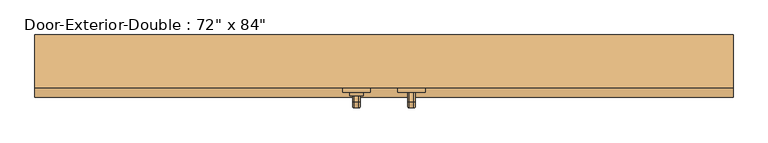
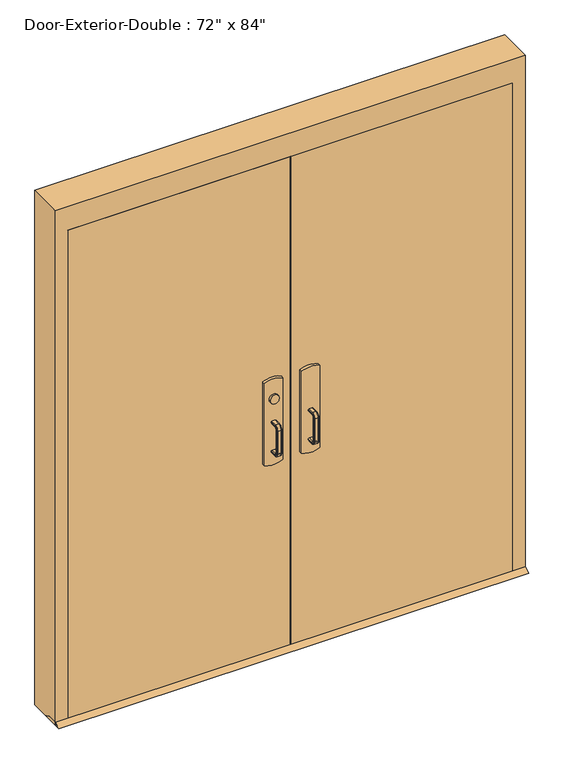
"""IFC4 building model written with IfcOpenShell, lengths in millimetres: door geometry."""

from ifc_helpers import new_model, si_unit, point, frame, frame_2d, origin, place, context, project, spatial, polyline, circle_curve, ellipse_curve, trimmed, segment, composite_curve, outline, extrude, faceted_brep, source, transform, mapped, element, save
from ifc_brep_helpers import plane_surface, cylinder_surface, revolved_surface, advanced_brep


def door_c6cb3189(model_context):
    return source(origin(), model_context, "Body", "SolidModel", [
        extrude(outline(polyline([(-575.7333333, 12.7), (-76.2, 12.7), (-76.2, 6.35), (-575.7333333, 6.35), (-575.7333333, 12.7)])), frame((0.0, 0.0, 990.6), z_axis=(0.0, 0.0, 1.0), x_axis=(1.0, 0.0, 0.0)), (0.0, 0.0, 1.0), 50.8),
        advanced_brep(
        [(-12.7, 6.35, 1041.4), (-12.7, 6.35, 990.6), (-76.2, 6.35, 990.6), (-825.5, 6.35, 990.6), (-825.5, 6.35, 1041.4), (-76.2, 6.35, 1041.4), (-825.5, -25.4, 1041.4), (-825.5, -25.4, 990.6), (-76.2, -25.4, 990.6), (-76.2, -25.4, 927.1), (-57.15, -25.4, 908.05), (-31.75, -25.4, 908.05), (-12.7, -25.4, 927.1), (-12.7, -25.4, 1104.9), (-31.75, -25.4, 1123.95), (-57.15, -25.4, 1123.95), (-76.2, -25.4, 1104.9), (-76.2, -25.4, 1041.4), (-76.2, 3.1747533, 1041.4), (-12.7, 3.1747533, 1041.4), (-12.7, -1.8354269, 1104.9), (-12.7, -1.8354269, 927.1), (-12.7, 3.1747533, 990.6), (-76.2, 3.1747533, 990.6), (-76.2, -1.8354269, 1104.9), (-76.2, -1.8354269, 927.1), (-31.75, -3.338481, 1123.95), (-57.15, -3.338481, 1123.95), (-57.15, -3.338481, 908.05), (-31.75, -3.338481, 908.05)],
        [
            (0, 1),
            (1, 2),
            (2, 3),
            (3, 4),
            (4, 5),
            (5, 0),
            (6, 7),
            (7, 8),
            (8, 9),
            (9, 10, circle_curve(frame((-57.15, -25.4, 927.1), z_axis=(0.0, -1.0, 0.0), x_axis=(-1.0, 0.0, 0.0)), 19.05)),
            (10, 11),
            (11, 12, circle_curve(frame((-31.75, -25.4, 927.1), z_axis=(0.0, -1.0, 0.0), x_axis=(-1.0, 0.0, 0.0)), 19.05)),
            (12, 13),
            (13, 14, circle_curve(frame((-31.75, -25.4, 1104.9), z_axis=(0.0, -1.0, 0.0), x_axis=(-1.0, 0.0, 0.0)), 19.05)),
            (14, 15),
            (15, 16, circle_curve(frame((-57.15, -25.4, 1104.9), z_axis=(0.0, -1.0, 0.0), x_axis=(-1.0, 0.0, 0.0)), 19.05)),
            (16, 17),
            (17, 6),
            (4, 6),
            (17, 18),
            (18, 19),
            (19, 0),
            (19, 20),
            (20, 13),
            (12, 21),
            (21, 22),
            (22, 1),
            (7, 3),
            (22, 23),
            (23, 8),
            (16, 24),
            (24, 18),
            (23, 25),
            (25, 9),
            (14, 26),
            (26, 27),
            (27, 15),
            (10, 28),
            (28, 29),
            (29, 11),
            (25, 28, ellipse_curve(frame((-57.15, -1.8354269, 927.1), z_axis=(0.0, -0.9969018152893365, 0.07865602756830282), x_axis=(0.0, 0.07865602756830208, 0.9969018152893365)), 19.1092038, 19.05)),
            (27, 24, ellipse_curve(frame((-57.15, -1.8354269, 1104.9), z_axis=(0.0, -0.9969018152893376, -0.07865602756828934), x_axis=(0.0, 0.078656027568288, -0.9969018152893377)), 19.1092038, 19.05)),
            (20, 26, ellipse_curve(frame((-31.75, -1.8354269, 1104.9), z_axis=(0.0, -0.9969018152893376, -0.07865602756828934), x_axis=(0.0, 0.078656027568288, -0.9969018152893377)), 19.1092038, 19.05)),
            (29, 21, ellipse_curve(frame((-31.75, -1.8354269, 927.1), z_axis=(0.0, -0.9969018152893365, 0.07865602756830282), x_axis=(0.0, 0.07865602756830208, 0.9969018152893365)), 19.1092038, 19.05)),
        ],
        [
            plane_surface(frame((-12.7, 6.35, 1041.4), z_axis=(0.0, 1.0, 0.0), x_axis=(1.0, 0.0, 0.0))),
            plane_surface(frame((-12.7, -25.4, 1041.4), z_axis=(0.0, -1.0, 0.0), x_axis=(-1.0, 0.0, 0.0))),
            plane_surface(frame((-825.5, 6.35, 1041.4), z_axis=(0.0, 0.0, 1.0), x_axis=(0.0, -1.0, 0.0))),
            plane_surface(frame((-12.7, 6.35, 1041.4), z_axis=(1.0, 0.0, 0.0), x_axis=(0.0, -1.0, 0.0))),
            plane_surface(frame((-12.7, 6.35, 990.6), z_axis=(0.0, 0.0, -1.0), x_axis=(0.0, -1.0, 0.0))),
            plane_surface(frame((-825.5, 6.35, 990.6), z_axis=(-1.0, 0.0, 0.0), x_axis=(0.0, -1.0, 0.0))),
            plane_surface(frame((-76.2, 3.1747533, 927.1), z_axis=(-1.0, 0.0, 0.0), x_axis=(0.0, -1.0, 0.0))),
            plane_surface(frame((-57.15, 3.1747533, 1123.95), z_axis=(0.0, 0.0, 1.0), x_axis=(0.0, -1.0, 0.0))),
            plane_surface(frame((-31.75, 3.1747533, 908.05), z_axis=(0.0, 0.0, -1.0), x_axis=(0.0, -1.0, 0.0))),
            cylinder_surface(frame((-57.15, -25.4, 927.1), z_axis=(0.0, 1.0, 0.0), x_axis=(-1.0, 0.0, 0.0)), 19.05),
            cylinder_surface(frame((-57.15, -25.4, 1104.9), z_axis=(0.0, 1.0, 0.0), x_axis=(-1.0, 0.0, 0.0)), 19.05),
            cylinder_surface(frame((-31.75, -25.4, 1104.9), z_axis=(0.0, 1.0, 0.0), x_axis=(-1.0, 0.0, 0.0)), 19.05),
            cylinder_surface(frame((-31.75, -25.4, 927.1), z_axis=(0.0, 1.0, 0.0), x_axis=(-1.0, 0.0, 0.0)), 19.05),
            plane_surface(frame((-76.2, 3.1747533, 1041.4), z_axis=(0.0, 0.9969018152893376, 0.07865602756828934), x_axis=(1.0, 0.0, 0.0))),
            plane_surface(frame((-76.2, -3.338481, 908.05), z_axis=(0.0, 0.9969018152893365, -0.07865602756830282), x_axis=(1.0, 0.0, 0.0))),
        ],
        [
            (0, [[1, 2, 3, 4, 5, 6]]),
            (1, [[7, 8, 9, 10, 11, 12, 13, 14, 15, 16, 17, 18]]),
            (2, [[19, -18, 20, 21, 22, -6, -5]]),
            (3, [[-1, -22, 23, 24, -13, 25, 26, 27]]),
            (4, [[28, -3, -2, -27, 29, 30, -8]]),
            (5, [[-4, -28, -7, -19]]),
            (6, [[-17, 31, 32, -20]]),
            (6, [[-9, -30, 33, 34]]),
            (7, [[-15, 35, 36, 37]]),
            (8, [[-11, 38, 39, 40]]),
            (9, [[-10, -34, 41, -38]]),
            (10, [[-16, -37, 42, -31]]),
            (11, [[-14, -24, 43, -35]]),
            (12, [[-12, -40, 44, -25]]),
            (13, [[-21, -32, -42, -36, -43, -23]]),
            (14, [[-26, -44, -39, -41, -33, -29]]),
        ],
    ),
        extrude(outline(polyline([(-69.85, 12.7), (-25.4, 12.7), (0.0, 0.0), (-95.25, 0.0), (-69.85, 12.7)])), frame((-965.2, 0.0, 0.0), z_axis=(1.0, 0.0, 0.0), x_axis=(0.0, 1.0, 0.0)), (0.0, 0.0, 1.0), 1930.4),
        extrude(outline(polyline([(575.7333333, 12.7), (575.7333333, 6.35), (76.2, 6.35), (76.2, 12.7), (575.7333333, 12.7)])), frame((0.0, 0.0, 990.6), z_axis=(0.0, 0.0, 1.0), x_axis=(1.0, 0.0, 0.0)), (0.0, 0.0, 1.0), 50.8),
        advanced_brep(
        [(12.7, 6.35, 1041.4), (76.2, 6.35, 1041.4), (825.5, 6.35, 1041.4), (825.5, 6.35, 990.6), (76.2, 6.35, 990.6), (12.7, 6.35, 990.6), (825.5, -25.4, 1041.4), (76.2, -25.4, 1041.4), (76.2, -25.4, 1104.9), (57.15, -25.4, 1123.95), (31.75, -25.4, 1123.95), (12.7, -25.4, 1104.9), (12.7, -25.4, 927.1), (31.75, -25.4, 908.05), (57.15, -25.4, 908.05), (76.2, -25.4, 927.1), (76.2, -25.4, 990.6), (825.5, -25.4, 990.6), (12.7, 3.1747533, 1041.4), (76.2, 3.1747533, 1041.4), (12.7, 3.1747533, 990.6), (12.7, -1.8354269, 927.1), (12.7, -1.8354269, 1104.9), (76.2, 3.1747533, 990.6), (76.2, -1.8354269, 1104.9), (76.2, -1.8354269, 927.1), (57.15, -3.338481, 1123.95), (31.75, -3.338481, 1123.95), (31.75, -3.338481, 908.05), (57.15, -3.338481, 908.05)],
        [
            (0, 1),
            (1, 2),
            (2, 3),
            (3, 4),
            (4, 5),
            (5, 0),
            (6, 7),
            (7, 8),
            (8, 9, circle_curve(frame((57.15, -25.4, 1104.9), z_axis=(0.0, -1.0, 0.0), x_axis=(1.0, 0.0, 0.0)), 19.05)),
            (9, 10),
            (10, 11, circle_curve(frame((31.75, -25.4, 1104.9), z_axis=(0.0, -1.0, 0.0), x_axis=(1.0, 0.0, 0.0)), 19.05)),
            (11, 12),
            (12, 13, circle_curve(frame((31.75, -25.4, 927.1), z_axis=(0.0, -1.0, 0.0), x_axis=(1.0, 0.0, 0.0)), 19.05)),
            (13, 14),
            (14, 15, circle_curve(frame((57.15, -25.4, 927.1), z_axis=(0.0, -1.0, 0.0), x_axis=(1.0, 0.0, 0.0)), 19.05)),
            (15, 16),
            (16, 17),
            (17, 6),
            (0, 18),
            (18, 19),
            (19, 7),
            (6, 2),
            (5, 20),
            (20, 21),
            (21, 12),
            (11, 22),
            (22, 18),
            (16, 23),
            (23, 20),
            (3, 17),
            (19, 24),
            (24, 8),
            (15, 25),
            (25, 23),
            (9, 26),
            (26, 27),
            (27, 10),
            (13, 28),
            (28, 29),
            (29, 14),
            (29, 25, ellipse_curve(frame((57.15, -1.8354269, 927.1), z_axis=(0.0, -0.9969018152893365, 0.07865602756830282), x_axis=(0.0, 0.07865602756830208, 0.9969018152893365)), 19.1092038, 19.05)),
            (24, 26, ellipse_curve(frame((57.15, -1.8354269, 1104.9), z_axis=(0.0, -0.9969018152893376, -0.07865602756828934), x_axis=(0.0, 0.078656027568288, -0.9969018152893377)), 19.1092038, 19.05)),
            (27, 22, ellipse_curve(frame((31.75, -1.8354269, 1104.9), z_axis=(0.0, -0.9969018152893376, -0.07865602756828934), x_axis=(0.0, 0.078656027568288, -0.9969018152893377)), 19.1092038, 19.05)),
            (21, 28, ellipse_curve(frame((31.75, -1.8354269, 927.1), z_axis=(0.0, -0.9969018152893365, 0.07865602756830282), x_axis=(0.0, 0.07865602756830208, 0.9969018152893365)), 19.1092038, 19.05)),
        ],
        [
            plane_surface(frame((12.7, 6.35, 1041.4), z_axis=(0.0, 1.0, 0.0), x_axis=(-1.0, 0.0, 0.0))),
            plane_surface(frame((12.7, -25.4, 1041.4), z_axis=(0.0, -1.0, 0.0), x_axis=(1.0, 0.0, 0.0))),
            plane_surface(frame((825.5, 6.35, 1041.4), z_axis=(0.0, 0.0, 1.0), x_axis=(0.0, -1.0, 0.0))),
            plane_surface(frame((12.7, 6.35, 1041.4), z_axis=(-1.0, 0.0, 0.0), x_axis=(0.0, -1.0, 0.0))),
            plane_surface(frame((12.7, 6.35, 990.6), z_axis=(0.0, 0.0, -1.0), x_axis=(0.0, -1.0, 0.0))),
            plane_surface(frame((825.5, 6.35, 990.6), z_axis=(1.0, 0.0, 0.0), x_axis=(0.0, -1.0, 0.0))),
            plane_surface(frame((76.2, 3.1747533, 927.1), z_axis=(1.0, 0.0, 0.0), x_axis=(0.0, -1.0, 0.0))),
            plane_surface(frame((57.15, 3.1747533, 1123.95), z_axis=(0.0, 0.0, 1.0), x_axis=(0.0, -1.0, 0.0))),
            plane_surface(frame((31.75, 3.1747533, 908.05), z_axis=(0.0, 0.0, -1.0), x_axis=(0.0, -1.0, 0.0))),
            cylinder_surface(frame((57.15, -25.4, 927.1), z_axis=(0.0, 1.0, 0.0), x_axis=(1.0, 0.0, 0.0)), 19.05),
            cylinder_surface(frame((57.15, -25.4, 1104.9), z_axis=(0.0, 1.0, 0.0), x_axis=(1.0, 0.0, 0.0)), 19.05),
            cylinder_surface(frame((31.75, -25.4, 1104.9), z_axis=(0.0, 1.0, 0.0), x_axis=(1.0, 0.0, 0.0)), 19.05),
            cylinder_surface(frame((31.75, -25.4, 927.1), z_axis=(0.0, 1.0, 0.0), x_axis=(1.0, 0.0, 0.0)), 19.05),
            plane_surface(frame((76.2, 3.1747533, 1041.4), z_axis=(0.0, 0.9969018152893376, 0.07865602756828934), x_axis=(-1.0, 0.0, 0.0))),
            plane_surface(frame((76.2, -3.338481, 908.05), z_axis=(0.0, 0.9969018152893365, -0.07865602756830282), x_axis=(-1.0, 0.0, 0.0))),
        ],
        [
            (0, [[1, 2, 3, 4, 5, 6]]),
            (1, [[7, 8, 9, 10, 11, 12, 13, 14, 15, 16, 17, 18]]),
            (2, [[-2, -1, 19, 20, 21, -7, 22]]),
            (3, [[23, 24, 25, -12, 26, 27, -19, -6]]),
            (4, [[-17, 28, 29, -23, -5, -4, 30]]),
            (5, [[-22, -18, -30, -3]]),
            (6, [[-21, 31, 32, -8]]),
            (6, [[33, 34, -28, -16]]),
            (7, [[35, 36, 37, -10]]),
            (8, [[38, 39, 40, -14]]),
            (9, [[-40, 41, -33, -15]]),
            (10, [[-32, 42, -35, -9]]),
            (11, [[-37, 43, -26, -11]]),
            (12, [[-25, 44, -38, -13]]),
            (13, [[-27, -43, -36, -42, -31, -20]]),
            (14, [[-29, -34, -41, -39, -44, -24]]),
        ],
    ),
        advanced_brep(
        [(66.2, -82.55, 1017.190625), (69.771875, -82.55, 1020.7625), (82.628125, -82.55, 1020.7625), (86.2, -82.55, 1017.190625), (86.2, -82.55, 1014.8090406), (82.6284594, -82.55, 1011.2375), (69.771875, -82.55, 1011.2375), (66.2, -82.55, 1014.809375), (66.2, -82.55, 887.809375), (66.2, -82.55, 890.190625), (69.771875, -82.55, 893.7625), (82.6284594, -82.55, 893.7625), (86.2, -82.55, 890.1909594), (86.2, -82.55, 887.809375), (82.628125, -82.55, 884.2375), (69.771875, -82.55, 884.2375), (66.2, -107.95, 1014.809375), (66.2, -119.459375, 1003.3), (66.2, -119.459375, 901.7), (66.2, -107.95, 890.190625), (66.2, -107.95, 887.809375), (66.2, -121.840625, 901.7), (66.2, -121.840625, 1003.3), (66.2, -107.95, 1017.190625), (69.771875, -107.95, 1011.2375), (82.6284594, -107.95, 1011.2375), (86.2, -107.95, 1014.8090406), (86.2, -107.95, 1017.190625), (86.2, -121.840625, 1003.3), (86.2, -121.840625, 901.7), (86.2, -107.95, 887.809375), (86.2, -107.95, 890.1909594), (86.2, -119.4590406, 901.7), (86.2, -119.4590406, 1003.3), (82.628125, -107.95, 1020.7625), (69.771875, -107.95, 1020.7625), (69.771875, -115.8875, 1003.3), (82.6284594, -115.8875, 1003.3), (82.628125, -125.4125, 1003.3), (69.771875, -125.4125, 1003.3), (69.771875, -115.8875, 901.7), (82.6284594, -115.8875, 901.7), (82.628125, -125.4125, 901.7), (69.771875, -125.4125, 901.7), (69.771875, -107.95, 893.7625), (82.6284594, -107.95, 893.7625), (82.628125, -107.95, 884.2375), (69.771875, -107.95, 884.2375)],
        [
            (0, 1, circle_curve(frame((69.771875, -82.55, 1017.190625), z_axis=(0.0, 1.0, 0.0), x_axis=(0.0, 0.0, 1.0)), 3.571875)),
            (1, 2),
            (2, 3, circle_curve(frame((82.628125, -82.55, 1017.190625), z_axis=(0.0, 1.0, 0.0), x_axis=(0.0, 0.0, 1.0)), 3.571875)),
            (3, 4),
            (4, 5, circle_curve(frame((82.6284594, -82.55, 1014.8090406), z_axis=(0.0, 1.0, 0.0), x_axis=(0.0, 0.0, 1.0)), 3.5715406)),
            (5, 6),
            (6, 7, circle_curve(frame((69.771875, -82.55, 1014.809375), z_axis=(0.0, 1.0, 0.0), x_axis=(0.0, 0.0, 1.0)), 3.571875)),
            (7, 0),
            (8, 9),
            (9, 10, circle_curve(frame((69.771875, -82.55, 890.190625), z_axis=(0.0, 1.0, 0.0), x_axis=(0.0, 0.0, -1.0)), 3.571875)),
            (10, 11),
            (11, 12, circle_curve(frame((82.6284594, -82.55, 890.1909594), z_axis=(0.0, 1.0, 0.0), x_axis=(0.0, 0.0, -1.0)), 3.5715406)),
            (12, 13),
            (13, 14, circle_curve(frame((82.628125, -82.55, 887.809375), z_axis=(0.0, 1.0, 0.0), x_axis=(0.0, 0.0, -1.0)), 3.571875)),
            (14, 15),
            (15, 8, circle_curve(frame((69.771875, -82.55, 887.809375), z_axis=(0.0, 1.0, 0.0), x_axis=(0.0, 0.0, -1.0)), 3.571875)),
            (7, 16),
            (16, 17, circle_curve(frame((66.2, -107.95, 1003.3), z_axis=(1.0, 0.0, 0.0), x_axis=(0.0, 0.0, 1.0)), 11.509375)),
            (17, 18),
            (18, 19, circle_curve(frame((66.2, -107.95, 901.7), z_axis=(1.0, 0.0, 0.0), x_axis=(0.0, -1.0, 0.0)), 11.509375)),
            (19, 9),
            (8, 20),
            (20, 21, circle_curve(frame((66.2, -107.95, 901.7), z_axis=(-1.0, 0.0, 0.0), x_axis=(0.0, -1.0, 0.0)), 13.890625)),
            (21, 22),
            (22, 23, circle_curve(frame((66.2, -107.95, 1003.3), z_axis=(-1.0, 0.0, 0.0), x_axis=(0.0, 0.0, 1.0)), 13.890625)),
            (23, 0),
            (6, 24),
            (24, 16, circle_curve(frame((69.771875, -107.95, 1014.809375), z_axis=(0.0, 1.0, 0.0), x_axis=(0.0, 0.0, 1.0)), 3.571875)),
            (5, 25),
            (25, 24),
            (4, 26),
            (26, 25, circle_curve(frame((82.6284594, -107.95, 1014.8090406), z_axis=(0.0, 1.0, 0.0), x_axis=(0.0, 0.0, 1.0)), 3.5715406)),
            (3, 27),
            (27, 28, circle_curve(frame((86.2, -107.95, 1003.3), z_axis=(1.0, 0.0, 0.0), x_axis=(0.0, 0.0, 1.0)), 13.890625)),
            (28, 29),
            (29, 30, circle_curve(frame((86.2, -107.95, 901.7), z_axis=(1.0, 0.0, 0.0), x_axis=(0.0, -1.0, 0.0)), 13.890625)),
            (30, 13),
            (12, 31),
            (31, 32, circle_curve(frame((86.2, -107.95, 901.7), z_axis=(-1.0, 0.0, 0.0), x_axis=(0.0, -1.0, 0.0)), 11.5090406)),
            (32, 33),
            (33, 26, circle_curve(frame((86.2, -107.95, 1003.3), z_axis=(-1.0, 0.0, 0.0), x_axis=(0.0, 0.0, 1.0)), 11.5090406)),
            (2, 34),
            (34, 27, circle_curve(frame((82.628125, -107.95, 1017.190625), z_axis=(0.0, 1.0, 0.0), x_axis=(0.0, 0.0, 1.0)), 3.571875)),
            (1, 35),
            (35, 34),
            (23, 35, circle_curve(frame((69.771875, -107.95, 1017.190625), z_axis=(0.0, 1.0, 0.0), x_axis=(0.0, 0.0, 1.0)), 3.571875)),
            (36, 17, circle_curve(frame((69.771875, -119.459375, 1003.3), z_axis=(0.0, 0.0, 1.0), x_axis=(0.0, -1.0, 0.0)), 3.571875)),
            (24, 36, circle_curve(frame((69.771875, -107.95, 1003.3), z_axis=(1.0, 0.0, 0.0), x_axis=(0.0, 0.0, 1.0)), 7.9375)),
            (37, 36),
            (25, 37, circle_curve(frame((82.6284594, -107.95, 1003.3), z_axis=(1.0, 0.0, 0.0), x_axis=(0.0, 0.0, 1.0)), 7.9375)),
            (33, 37, circle_curve(frame((82.6284594, -119.4590406, 1003.3), z_axis=(0.0, 0.0, 1.0), x_axis=(0.0, -1.0, 0.0)), 3.5715406)),
            (38, 28, circle_curve(frame((82.628125, -121.840625, 1003.3), z_axis=(0.0, 0.0, 1.0), x_axis=(0.0, -1.0, 0.0)), 3.571875)),
            (34, 38, circle_curve(frame((82.628125, -107.95, 1003.3), z_axis=(1.0, 0.0, 0.0), x_axis=(0.0, 0.0, 1.0)), 17.4625)),
            (39, 38),
            (35, 39, circle_curve(frame((69.771875, -107.95, 1003.3), z_axis=(1.0, 0.0, 0.0), x_axis=(0.0, 0.0, 1.0)), 17.4625)),
            (22, 39, circle_curve(frame((69.771875, -121.840625, 1003.3), z_axis=(0.0, 0.0, 1.0), x_axis=(0.0, -1.0, 0.0)), 3.571875)),
            (36, 40),
            (40, 18, circle_curve(frame((69.771875, -119.459375, 901.7), z_axis=(0.0, 0.0, 1.0), x_axis=(0.0, -1.0, 0.0)), 3.571875)),
            (37, 41),
            (41, 40),
            (32, 41, circle_curve(frame((82.6284594, -119.4590406, 901.7), z_axis=(0.0, 0.0, 1.0), x_axis=(0.0, -1.0, 0.0)), 3.5715406)),
            (38, 42),
            (42, 29, circle_curve(frame((82.628125, -121.840625, 901.7), z_axis=(0.0, 0.0, 1.0), x_axis=(0.0, -1.0, 0.0)), 3.571875)),
            (39, 43),
            (43, 42),
            (21, 43, circle_curve(frame((69.771875, -121.840625, 901.7), z_axis=(0.0, 0.0, 1.0), x_axis=(0.0, -1.0, 0.0)), 3.571875)),
            (44, 19, circle_curve(frame((69.771875, -107.95, 890.190625), z_axis=(0.0, -1.0, 0.0), x_axis=(0.0, 0.0, -1.0)), 3.571875)),
            (40, 44, circle_curve(frame((69.771875, -107.95, 901.7), z_axis=(1.0, 0.0, 0.0), x_axis=(0.0, -1.0, 0.0)), 7.9375)),
            (45, 44),
            (41, 45, circle_curve(frame((82.6284594, -107.95, 901.7), z_axis=(1.0, 0.0, 0.0), x_axis=(0.0, -1.0, 0.0)), 7.9375)),
            (31, 45, circle_curve(frame((82.6284594, -107.95, 890.1909594), z_axis=(0.0, -1.0, 0.0), x_axis=(0.0, 0.0, -1.0)), 3.5715406)),
            (46, 30, circle_curve(frame((82.628125, -107.95, 887.809375), z_axis=(0.0, -1.0, 0.0), x_axis=(0.0, 0.0, -1.0)), 3.571875)),
            (42, 46, circle_curve(frame((82.628125, -107.95, 901.7), z_axis=(1.0, 0.0, 0.0), x_axis=(0.0, -1.0, 0.0)), 17.4625)),
            (47, 46),
            (43, 47, circle_curve(frame((69.771875, -107.95, 901.7), z_axis=(1.0, 0.0, 0.0), x_axis=(0.0, -1.0, 0.0)), 17.4625)),
            (20, 47, circle_curve(frame((69.771875, -107.95, 887.809375), z_axis=(0.0, -1.0, 0.0), x_axis=(0.0, 0.0, -1.0)), 3.571875)),
            (44, 10),
            (45, 11),
            (46, 14),
            (47, 15),
        ],
        [
            plane_surface(frame((76.2, -82.55, 1016.0), z_axis=(0.0, 1.0, 0.0), x_axis=(1.0, 0.0, 0.0))),
            plane_surface(frame((76.2, -82.55, 889.0), z_axis=(0.0, 1.0, 0.0), x_axis=(1.0, 0.0, 0.0))),
            plane_surface(frame((66.2, -82.55, 1017.190625), z_axis=(-1.0, 0.0, 0.0), x_axis=(0.0, -1.0, 0.0))),
            cylinder_surface(frame((69.771875, -82.55, 1014.809375), z_axis=(0.0, 1.0, 0.0), x_axis=(0.0, 0.0, 1.0)), 3.571875),
            plane_surface(frame((69.771875, -82.55, 1011.2375), z_axis=(0.0, 0.0, -1.0), x_axis=(0.0, -1.0, 0.0))),
            cylinder_surface(frame((82.6284594, -82.55, 1014.8090406), z_axis=(0.0, 1.0, 0.0), x_axis=(0.0, 0.0, 1.0)), 3.5715406),
            plane_surface(frame((86.2, -82.55, 1014.8090406), z_axis=(1.0, 0.0, 0.0), x_axis=(0.0, -1.0, 0.0))),
            cylinder_surface(frame((82.628125, -82.55, 1017.190625), z_axis=(0.0, 1.0, 0.0), x_axis=(0.0, 0.0, 1.0)), 3.571875),
            plane_surface(frame((82.628125, -82.55, 1020.7625), z_axis=(0.0, 0.0, 1.0), x_axis=(0.0, -1.0, 0.0))),
            cylinder_surface(frame((69.771875, -82.55, 1017.190625), z_axis=(0.0, 1.0, 0.0), x_axis=(0.0, 0.0, 1.0)), 3.571875),
            revolved_surface(trimmed(ellipse_curve(frame((69.771875, -107.95, 1014.809375), z_axis=(0.0, -1.0, 0.0), x_axis=(0.0, 0.0, 1.0)), 3.571875, 3.571875), [point((66.2, -107.95, 1014.809375))], [point((69.771875, -107.95, 1011.2375))], True, "CARTESIAN"), (76.2, -107.95, 1003.3), (-1.0, 0.0, 0.0)),
            revolved_surface(polyline([(69.771875, -107.95, 1011.2375), (82.6284594, -107.95, 1011.2375)]), (76.2, -107.95, 1003.3), (-1.0, 0.0, 0.0)),
            revolved_surface(trimmed(ellipse_curve(frame((82.6284594, -107.95, 1014.8090406), z_axis=(0.0, -1.0, 0.0), x_axis=(0.0, 0.0, 1.0)), 3.5715406, 3.5715406), [point((82.6284594, -107.95, 1011.2375))], [point((86.2, -107.95, 1014.8090406))], True, "CARTESIAN"), (76.2, -107.95, 1003.3), (-1.0, 0.0, 0.0)),
            revolved_surface(trimmed(ellipse_curve(frame((82.628125, -107.95, 1017.190625), z_axis=(0.0, -1.0, 0.0), x_axis=(0.0, 0.0, 1.0)), 3.571875, 3.571875), [point((86.2, -107.95, 1017.190625))], [point((82.628125, -107.95, 1020.7625))], True, "CARTESIAN"), (76.2, -107.95, 1003.3), (-1.0, 0.0, 0.0)),
            cylinder_surface(frame((76.2, -107.95, 1003.3), z_axis=(-1.0, 0.0, 0.0), x_axis=(0.0, 0.0, 1.0)), 17.4625),
            revolved_surface(trimmed(ellipse_curve(frame((69.771875, -107.95, 1017.190625), z_axis=(0.0, -1.0, 0.0), x_axis=(0.0, 0.0, 1.0)), 3.571875, 3.571875), [point((69.771875, -107.95, 1020.7625))], [point((66.2, -107.95, 1017.190625))], True, "CARTESIAN"), (76.2, -107.95, 1003.3), (-1.0, 0.0, 0.0)),
            cylinder_surface(frame((69.771875, -119.459375, 1003.3), z_axis=(0.0, 0.0, 1.0), x_axis=(0.0, -1.0, 0.0)), 3.571875),
            plane_surface(frame((69.771875, -115.8875, 1003.3), z_axis=(0.0, 1.0, 0.0), x_axis=(0.0, 0.0, -1.0))),
            cylinder_surface(frame((82.6284594, -119.4590406, 1003.3), z_axis=(0.0, 0.0, 1.0), x_axis=(0.0, -1.0, 0.0)), 3.5715406),
            cylinder_surface(frame((82.628125, -121.840625, 1003.3), z_axis=(0.0, 0.0, 1.0), x_axis=(0.0, -1.0, 0.0)), 3.571875),
            plane_surface(frame((82.628125, -125.4125, 1003.3), z_axis=(0.0, -1.0, 0.0), x_axis=(0.0, 0.0, -1.0))),
            cylinder_surface(frame((69.771875, -121.840625, 1003.3), z_axis=(0.0, 0.0, 1.0), x_axis=(0.0, -1.0, 0.0)), 3.571875),
            revolved_surface(trimmed(ellipse_curve(frame((69.771875, -119.459375, 901.7), z_axis=(0.0, 0.0, -1.0), x_axis=(0.0, -1.0, 0.0)), 3.571875, 3.571875), [point((66.2, -119.459375, 901.7))], [point((69.771875, -115.8875, 901.7))], True, "CARTESIAN"), (76.2, -107.95, 901.7), (-1.0, 0.0, 0.0)),
            revolved_surface(polyline([(69.771875, -115.8875, 901.7), (82.6284594, -115.8875, 901.7)]), (76.2, -107.95, 901.7), (-1.0, 0.0, 0.0)),
            revolved_surface(trimmed(ellipse_curve(frame((82.6284594, -119.4590406, 901.7), z_axis=(0.0, 0.0, -1.0), x_axis=(0.0, -1.0, 0.0)), 3.5715406, 3.5715406), [point((82.6284594, -115.8875, 901.7))], [point((86.2, -119.4590406, 901.7))], True, "CARTESIAN"), (76.2, -107.95, 901.7), (-1.0, 0.0, 0.0)),
            revolved_surface(trimmed(ellipse_curve(frame((82.628125, -121.840625, 901.7), z_axis=(0.0, 0.0, -1.0), x_axis=(0.0, -1.0, 0.0)), 3.571875, 3.571875), [point((86.2, -121.840625, 901.7))], [point((82.628125, -125.4125, 901.7))], True, "CARTESIAN"), (76.2, -107.95, 901.7), (-1.0, 0.0, 0.0)),
            cylinder_surface(frame((76.2, -107.95, 901.7), z_axis=(-1.0, 0.0, 0.0), x_axis=(0.0, -1.0, 0.0)), 17.4625),
            revolved_surface(trimmed(ellipse_curve(frame((69.771875, -121.840625, 901.7), z_axis=(0.0, 0.0, -1.0), x_axis=(0.0, -1.0, 0.0)), 3.571875, 3.571875), [point((69.771875, -125.4125, 901.7))], [point((66.2, -121.840625, 901.7))], True, "CARTESIAN"), (76.2, -107.95, 901.7), (-1.0, 0.0, 0.0)),
            cylinder_surface(frame((69.771875, -107.95, 890.190625), z_axis=(0.0, -1.0, 0.0), x_axis=(0.0, 0.0, -1.0)), 3.571875),
            plane_surface(frame((69.771875, -107.95, 893.7625), z_axis=(0.0, 0.0, 1.0), x_axis=(0.0, 1.0, 0.0))),
            cylinder_surface(frame((82.6284594, -107.95, 890.1909594), z_axis=(0.0, -1.0, 0.0), x_axis=(0.0, 0.0, -1.0)), 3.5715406),
            cylinder_surface(frame((82.628125, -107.95, 887.809375), z_axis=(0.0, -1.0, 0.0), x_axis=(0.0, 0.0, -1.0)), 3.571875),
            plane_surface(frame((82.628125, -107.95, 884.2375), z_axis=(0.0, 0.0, -1.0), x_axis=(0.0, 1.0, 0.0))),
            cylinder_surface(frame((69.771875, -107.95, 887.809375), z_axis=(0.0, -1.0, 0.0), x_axis=(0.0, 0.0, -1.0)), 3.571875),
        ],
        [
            (0, [[1, 2, 3, 4, 5, 6, 7, 8]]),
            (1, [[9, 10, 11, 12, 13, 14, 15, 16]]),
            (2, [[17, 18, 19, 20, 21, -9, 22, 23, 24, 25, 26, -8]]),
            (3, [[27, 28, -17, -7]]),
            (4, [[29, 30, -27, -6]]),
            (5, [[31, 32, -29, -5]]),
            (6, [[33, 34, 35, 36, 37, -13, 38, 39, 40, 41, -31, -4]]),
            (7, [[42, 43, -33, -3]]),
            (8, [[44, 45, -42, -2]]),
            (9, [[-26, 46, -44, -1]]),
            (10, [[47, -18, -28, 48]]),
            (11, [[49, -48, -30, 50]]),
            (12, [[51, -50, -32, -41]]),
            (13, [[52, -34, -43, 53]]),
            (14, [[54, -53, -45, 55]]),
            (15, [[56, -55, -46, -25]]),
            (16, [[57, 58, -19, -47]]),
            (17, [[59, 60, -57, -49]]),
            (18, [[-40, 61, -59, -51]]),
            (19, [[62, 63, -35, -52]]),
            (20, [[64, 65, -62, -54]]),
            (21, [[-24, 66, -64, -56]]),
            (22, [[67, -20, -58, 68]]),
            (23, [[69, -68, -60, 70]]),
            (24, [[71, -70, -61, -39]]),
            (25, [[72, -36, -63, 73]]),
            (26, [[74, -73, -65, 75]]),
            (27, [[76, -75, -66, -23]]),
            (28, [[77, -10, -21, -67]]),
            (29, [[78, -11, -77, -69]]),
            (30, [[-38, -12, -78, -71]]),
            (31, [[79, -14, -37, -72]]),
            (32, [[80, -15, -79, -74]]),
            (33, [[-22, -16, -80, -76]]),
        ],
    ),
        extrude(outline(composite_curve([segment(trimmed(circle_curve(frame_2d((1113.0338574, 76.2)), 89.3016225), [point((1193.8, 114.3))], [point((1193.8, 38.1))], False, "CARTESIAN"), True, "CONTINUOUS"), segment(polyline([(1193.8, 38.1), (838.2, 38.1)]), True, "CONTINUOUS"), segment(trimmed(circle_curve(frame_2d((918.9661426, 76.2)), 89.3016225), [point((838.2, 38.1))], [point((838.2, 114.3))], False, "CARTESIAN"), True, "CONTINUOUS"), segment(polyline([(838.2, 114.3), (1193.8, 114.3)]), True, "CONTINUOUS")], self_intersect=False)), frame((0.0, -82.55, 0.0), z_axis=(0.0, 1.0, 0.0), x_axis=(0.0, 0.0, 1.0)), (0.0, 0.0, 1.0), 12.7),
        advanced_brep(
        [(-86.2, -82.55, 1017.190625), (-82.628125, -82.55, 1020.7625), (-69.771875, -82.55, 1020.7625), (-66.2, -82.55, 1017.190625), (-66.2, -82.55, 1014.8090406), (-69.7715406, -82.55, 1011.2375), (-82.628125, -82.55, 1011.2375), (-86.2, -82.55, 1014.809375), (-86.2, -82.55, 887.809375), (-86.2, -82.55, 890.190625), (-82.628125, -82.55, 893.7625), (-69.7715406, -82.55, 893.7625), (-66.2, -82.55, 890.1909594), (-66.2, -82.55, 887.809375), (-69.771875, -82.55, 884.2375), (-82.628125, -82.55, 884.2375), (-86.2, -107.95, 1014.809375), (-86.2, -119.459375, 1003.3), (-86.2, -119.459375, 901.7), (-86.2, -107.95, 890.190625), (-86.2, -107.95, 887.809375), (-86.2, -121.840625, 901.7), (-86.2, -121.840625, 1003.3), (-86.2, -107.95, 1017.190625), (-82.628125, -107.95, 1011.2375), (-69.7715406, -107.95, 1011.2375), (-66.2, -107.95, 1014.8090406), (-66.2, -107.95, 1017.190625), (-66.2, -121.840625, 1003.3), (-66.2, -121.840625, 901.7), (-66.2, -107.95, 887.809375), (-66.2, -107.95, 890.1909594), (-66.2, -119.4590406, 901.7), (-66.2, -119.4590406, 1003.3), (-69.771875, -107.95, 1020.7625), (-82.628125, -107.95, 1020.7625), (-82.628125, -115.8875, 1003.3), (-69.7715406, -115.8875, 1003.3), (-69.771875, -125.4125, 1003.3), (-82.628125, -125.4125, 1003.3), (-82.628125, -115.8875, 901.7), (-69.7715406, -115.8875, 901.7), (-69.771875, -125.4125, 901.7), (-82.628125, -125.4125, 901.7), (-82.628125, -107.95, 893.7625), (-69.7715406, -107.95, 893.7625), (-69.771875, -107.95, 884.2375), (-82.628125, -107.95, 884.2375)],
        [
            (0, 1, circle_curve(frame((-82.628125, -82.55, 1017.190625), z_axis=(0.0, 1.0, 0.0), x_axis=(0.0, 0.0, 1.0)), 3.571875)),
            (1, 2),
            (2, 3, circle_curve(frame((-69.771875, -82.55, 1017.190625), z_axis=(0.0, 1.0, 0.0), x_axis=(0.0, 0.0, 1.0)), 3.571875)),
            (3, 4),
            (4, 5, circle_curve(frame((-69.7715406, -82.55, 1014.8090406), z_axis=(0.0, 1.0, 0.0), x_axis=(0.0, 0.0, 1.0)), 3.5715406)),
            (5, 6),
            (6, 7, circle_curve(frame((-82.628125, -82.55, 1014.809375), z_axis=(0.0, 1.0, 0.0), x_axis=(0.0, 0.0, 1.0)), 3.571875)),
            (7, 0),
            (8, 9),
            (9, 10, circle_curve(frame((-82.628125, -82.55, 890.190625), z_axis=(0.0, 1.0, 0.0), x_axis=(0.0, 0.0, -1.0)), 3.571875)),
            (10, 11),
            (11, 12, circle_curve(frame((-69.7715406, -82.55, 890.1909594), z_axis=(0.0, 1.0, 0.0), x_axis=(0.0, 0.0, -1.0)), 3.5715406)),
            (12, 13),
            (13, 14, circle_curve(frame((-69.771875, -82.55, 887.809375), z_axis=(0.0, 1.0, 0.0), x_axis=(0.0, 0.0, -1.0)), 3.571875)),
            (14, 15),
            (15, 8, circle_curve(frame((-82.628125, -82.55, 887.809375), z_axis=(0.0, 1.0, 0.0), x_axis=(0.0, 0.0, -1.0)), 3.571875)),
            (7, 16),
            (16, 17, circle_curve(frame((-86.2, -107.95, 1003.3), z_axis=(1.0, 0.0, 0.0), x_axis=(0.0, 0.0, 1.0)), 11.509375)),
            (17, 18),
            (18, 19, circle_curve(frame((-86.2, -107.95, 901.7), z_axis=(1.0, 0.0, 0.0), x_axis=(0.0, -1.0, 0.0)), 11.509375)),
            (19, 9),
            (8, 20),
            (20, 21, circle_curve(frame((-86.2, -107.95, 901.7), z_axis=(-1.0, 0.0, 0.0), x_axis=(0.0, -1.0, 0.0)), 13.890625)),
            (21, 22),
            (22, 23, circle_curve(frame((-86.2, -107.95, 1003.3), z_axis=(-1.0, 0.0, 0.0), x_axis=(0.0, 0.0, 1.0)), 13.890625)),
            (23, 0),
            (6, 24),
            (24, 16, circle_curve(frame((-82.628125, -107.95, 1014.809375), z_axis=(0.0, 1.0, 0.0), x_axis=(0.0, 0.0, 1.0)), 3.571875)),
            (5, 25),
            (25, 24),
            (4, 26),
            (26, 25, circle_curve(frame((-69.7715406, -107.95, 1014.8090406), z_axis=(0.0, 1.0, 0.0), x_axis=(0.0, 0.0, 1.0)), 3.5715406)),
            (3, 27),
            (27, 28, circle_curve(frame((-66.2, -107.95, 1003.3), z_axis=(1.0, 0.0, 0.0), x_axis=(0.0, 0.0, 1.0)), 13.890625)),
            (28, 29),
            (29, 30, circle_curve(frame((-66.2, -107.95, 901.7), z_axis=(1.0, 0.0, 0.0), x_axis=(0.0, -1.0, 0.0)), 13.890625)),
            (30, 13),
            (12, 31),
            (31, 32, circle_curve(frame((-66.2, -107.95, 901.7), z_axis=(-1.0, 0.0, 0.0), x_axis=(0.0, -1.0, 0.0)), 11.5090406)),
            (32, 33),
            (33, 26, circle_curve(frame((-66.2, -107.95, 1003.3), z_axis=(-1.0, 0.0, 0.0), x_axis=(0.0, 0.0, 1.0)), 11.5090406)),
            (2, 34),
            (34, 27, circle_curve(frame((-69.771875, -107.95, 1017.190625), z_axis=(0.0, 1.0, 0.0), x_axis=(0.0, 0.0, 1.0)), 3.571875)),
            (1, 35),
            (35, 34),
            (23, 35, circle_curve(frame((-82.628125, -107.95, 1017.190625), z_axis=(0.0, 1.0, 0.0), x_axis=(0.0, 0.0, 1.0)), 3.571875)),
            (36, 17, circle_curve(frame((-82.628125, -119.459375, 1003.3), z_axis=(0.0, 0.0, 1.0), x_axis=(0.0, -1.0, 0.0)), 3.571875)),
            (24, 36, circle_curve(frame((-82.628125, -107.95, 1003.3), z_axis=(1.0, 0.0, 0.0), x_axis=(0.0, 0.0, 1.0)), 7.9375)),
            (37, 36),
            (25, 37, circle_curve(frame((-69.7715406, -107.95, 1003.3), z_axis=(1.0, 0.0, 0.0), x_axis=(0.0, 0.0, 1.0)), 7.9375)),
            (33, 37, circle_curve(frame((-69.7715406, -119.4590406, 1003.3), z_axis=(0.0, 0.0, 1.0), x_axis=(0.0, -1.0, 0.0)), 3.5715406)),
            (38, 28, circle_curve(frame((-69.771875, -121.840625, 1003.3), z_axis=(0.0, 0.0, 1.0), x_axis=(0.0, -1.0, 0.0)), 3.571875)),
            (34, 38, circle_curve(frame((-69.771875, -107.95, 1003.3), z_axis=(1.0, 0.0, 0.0), x_axis=(0.0, 0.0, 1.0)), 17.4625)),
            (39, 38),
            (35, 39, circle_curve(frame((-82.628125, -107.95, 1003.3), z_axis=(1.0, 0.0, 0.0), x_axis=(0.0, 0.0, 1.0)), 17.4625)),
            (22, 39, circle_curve(frame((-82.628125, -121.840625, 1003.3), z_axis=(0.0, 0.0, 1.0), x_axis=(0.0, -1.0, 0.0)), 3.571875)),
            (36, 40),
            (40, 18, circle_curve(frame((-82.628125, -119.459375, 901.7), z_axis=(0.0, 0.0, 1.0), x_axis=(0.0, -1.0, 0.0)), 3.571875)),
            (37, 41),
            (41, 40),
            (32, 41, circle_curve(frame((-69.7715406, -119.4590406, 901.7), z_axis=(0.0, 0.0, 1.0), x_axis=(0.0, -1.0, 0.0)), 3.5715406)),
            (38, 42),
            (42, 29, circle_curve(frame((-69.771875, -121.840625, 901.7), z_axis=(0.0, 0.0, 1.0), x_axis=(0.0, -1.0, 0.0)), 3.571875)),
            (39, 43),
            (43, 42),
            (21, 43, circle_curve(frame((-82.628125, -121.840625, 901.7), z_axis=(0.0, 0.0, 1.0), x_axis=(0.0, -1.0, 0.0)), 3.571875)),
            (44, 19, circle_curve(frame((-82.628125, -107.95, 890.190625), z_axis=(0.0, -1.0, 0.0), x_axis=(0.0, 0.0, -1.0)), 3.571875)),
            (40, 44, circle_curve(frame((-82.628125, -107.95, 901.7), z_axis=(1.0, 0.0, 0.0), x_axis=(0.0, -1.0, 0.0)), 7.9375)),
            (45, 44),
            (41, 45, circle_curve(frame((-69.7715406, -107.95, 901.7), z_axis=(1.0, 0.0, 0.0), x_axis=(0.0, -1.0, 0.0)), 7.9375)),
            (31, 45, circle_curve(frame((-69.7715406, -107.95, 890.1909594), z_axis=(0.0, -1.0, 0.0), x_axis=(0.0, 0.0, -1.0)), 3.5715406)),
            (46, 30, circle_curve(frame((-69.771875, -107.95, 887.809375), z_axis=(0.0, -1.0, 0.0), x_axis=(0.0, 0.0, -1.0)), 3.571875)),
            (42, 46, circle_curve(frame((-69.771875, -107.95, 901.7), z_axis=(1.0, 0.0, 0.0), x_axis=(0.0, -1.0, 0.0)), 17.4625)),
            (47, 46),
            (43, 47, circle_curve(frame((-82.628125, -107.95, 901.7), z_axis=(1.0, 0.0, 0.0), x_axis=(0.0, -1.0, 0.0)), 17.4625)),
            (20, 47, circle_curve(frame((-82.628125, -107.95, 887.809375), z_axis=(0.0, -1.0, 0.0), x_axis=(0.0, 0.0, -1.0)), 3.571875)),
            (44, 10),
            (45, 11),
            (46, 14),
            (47, 15),
        ],
        [
            plane_surface(frame((-76.2, -82.55, 1016.0), z_axis=(0.0, 1.0, 0.0), x_axis=(1.0, 0.0, 0.0))),
            plane_surface(frame((-76.2, -82.55, 889.0), z_axis=(0.0, 1.0, 0.0), x_axis=(1.0, 0.0, 0.0))),
            plane_surface(frame((-86.2, -82.55, 1017.190625), z_axis=(-1.0, 0.0, 0.0), x_axis=(0.0, -1.0, 0.0))),
            cylinder_surface(frame((-82.628125, -82.55, 1014.809375), z_axis=(0.0, 1.0, 0.0), x_axis=(0.0, 0.0, 1.0)), 3.571875),
            plane_surface(frame((-82.628125, -82.55, 1011.2375), z_axis=(0.0, 0.0, -1.0), x_axis=(0.0, -1.0, 0.0))),
            cylinder_surface(frame((-69.7715406, -82.55, 1014.8090406), z_axis=(0.0, 1.0, 0.0), x_axis=(0.0, 0.0, 1.0)), 3.5715406),
            plane_surface(frame((-66.2, -82.55, 1014.8090406), z_axis=(1.0, 0.0, 0.0), x_axis=(0.0, -1.0, 0.0))),
            cylinder_surface(frame((-69.771875, -82.55, 1017.190625), z_axis=(0.0, 1.0, 0.0), x_axis=(0.0, 0.0, 1.0)), 3.571875),
            plane_surface(frame((-69.771875, -82.55, 1020.7625), z_axis=(0.0, 0.0, 1.0), x_axis=(0.0, -1.0, 0.0))),
            cylinder_surface(frame((-82.628125, -82.55, 1017.190625), z_axis=(0.0, 1.0, 0.0), x_axis=(0.0, 0.0, 1.0)), 3.571875),
            revolved_surface(trimmed(ellipse_curve(frame((-82.628125, -107.95, 1014.809375), z_axis=(0.0, -1.0, 0.0), x_axis=(0.0, 0.0, 1.0)), 3.571875, 3.571875), [point((-86.2, -107.95, 1014.809375))], [point((-82.628125, -107.95, 1011.2375))], True, "CARTESIAN"), (-76.2, -107.95, 1003.3), (-1.0, 0.0, 0.0)),
            revolved_surface(polyline([(-82.628125, -107.95, 1011.2375), (-69.7715406, -107.95, 1011.2375)]), (-76.2, -107.95, 1003.3), (-1.0, 0.0, 0.0)),
            revolved_surface(trimmed(ellipse_curve(frame((-69.7715406, -107.95, 1014.8090406), z_axis=(0.0, -1.0, 0.0), x_axis=(0.0, 0.0, 1.0)), 3.5715406, 3.5715406), [point((-69.7715406, -107.95, 1011.2375))], [point((-66.2, -107.95, 1014.8090406))], True, "CARTESIAN"), (-76.2, -107.95, 1003.3), (-1.0, 0.0, 0.0)),
            revolved_surface(trimmed(ellipse_curve(frame((-69.771875, -107.95, 1017.190625), z_axis=(0.0, -1.0, 0.0), x_axis=(0.0, 0.0, 1.0)), 3.571875, 3.571875), [point((-66.2, -107.95, 1017.190625))], [point((-69.771875, -107.95, 1020.7625))], True, "CARTESIAN"), (-76.2, -107.95, 1003.3), (-1.0, 0.0, 0.0)),
            cylinder_surface(frame((-76.2, -107.95, 1003.3), z_axis=(-1.0, 0.0, 0.0), x_axis=(0.0, 0.0, 1.0)), 17.4625),
            revolved_surface(trimmed(ellipse_curve(frame((-82.628125, -107.95, 1017.190625), z_axis=(0.0, -1.0, 0.0), x_axis=(0.0, 0.0, 1.0)), 3.571875, 3.571875), [point((-82.628125, -107.95, 1020.7625))], [point((-86.2, -107.95, 1017.190625))], True, "CARTESIAN"), (-76.2, -107.95, 1003.3), (-1.0, 0.0, 0.0)),
            cylinder_surface(frame((-82.628125, -119.459375, 1003.3), z_axis=(0.0, 0.0, 1.0), x_axis=(0.0, -1.0, 0.0)), 3.571875),
            plane_surface(frame((-82.628125, -115.8875, 1003.3), z_axis=(0.0, 1.0, 0.0), x_axis=(0.0, 0.0, -1.0))),
            cylinder_surface(frame((-69.7715406, -119.4590406, 1003.3), z_axis=(0.0, 0.0, 1.0), x_axis=(0.0, -1.0, 0.0)), 3.5715406),
            cylinder_surface(frame((-69.771875, -121.840625, 1003.3), z_axis=(0.0, 0.0, 1.0), x_axis=(0.0, -1.0, 0.0)), 3.571875),
            plane_surface(frame((-69.771875, -125.4125, 1003.3), z_axis=(0.0, -1.0, 0.0), x_axis=(0.0, 0.0, -1.0))),
            cylinder_surface(frame((-82.628125, -121.840625, 1003.3), z_axis=(0.0, 0.0, 1.0), x_axis=(0.0, -1.0, 0.0)), 3.571875),
            revolved_surface(trimmed(ellipse_curve(frame((-82.628125, -119.459375, 901.7), z_axis=(0.0, 0.0, -1.0), x_axis=(0.0, -1.0, 0.0)), 3.571875, 3.571875), [point((-86.2, -119.459375, 901.7))], [point((-82.628125, -115.8875, 901.7))], True, "CARTESIAN"), (-76.2, -107.95, 901.7), (-1.0, 0.0, 0.0)),
            revolved_surface(polyline([(-82.628125, -115.8875, 901.7), (-69.7715406, -115.8875, 901.7)]), (-76.2, -107.95, 901.7), (-1.0, 0.0, 0.0)),
            revolved_surface(trimmed(ellipse_curve(frame((-69.7715406, -119.4590406, 901.7), z_axis=(0.0, 0.0, -1.0), x_axis=(0.0, -1.0, 0.0)), 3.5715406, 3.5715406), [point((-69.7715406, -115.8875, 901.7))], [point((-66.2, -119.4590406, 901.7))], True, "CARTESIAN"), (-76.2, -107.95, 901.7), (-1.0, 0.0, 0.0)),
            revolved_surface(trimmed(ellipse_curve(frame((-69.771875, -121.840625, 901.7), z_axis=(0.0, 0.0, -1.0), x_axis=(0.0, -1.0, 0.0)), 3.571875, 3.571875), [point((-66.2, -121.840625, 901.7))], [point((-69.771875, -125.4125, 901.7))], True, "CARTESIAN"), (-76.2, -107.95, 901.7), (-1.0, 0.0, 0.0)),
            cylinder_surface(frame((-76.2, -107.95, 901.7), z_axis=(-1.0, 0.0, 0.0), x_axis=(0.0, -1.0, 0.0)), 17.4625),
            revolved_surface(trimmed(ellipse_curve(frame((-82.628125, -121.840625, 901.7), z_axis=(0.0, 0.0, -1.0), x_axis=(0.0, -1.0, 0.0)), 3.571875, 3.571875), [point((-82.628125, -125.4125, 901.7))], [point((-86.2, -121.840625, 901.7))], True, "CARTESIAN"), (-76.2, -107.95, 901.7), (-1.0, 0.0, 0.0)),
            cylinder_surface(frame((-82.628125, -107.95, 890.190625), z_axis=(0.0, -1.0, 0.0), x_axis=(0.0, 0.0, -1.0)), 3.571875),
            plane_surface(frame((-82.628125, -107.95, 893.7625), z_axis=(0.0, 0.0, 1.0), x_axis=(0.0, 1.0, 0.0))),
            cylinder_surface(frame((-69.7715406, -107.95, 890.1909594), z_axis=(0.0, -1.0, 0.0), x_axis=(0.0, 0.0, -1.0)), 3.5715406),
            cylinder_surface(frame((-69.771875, -107.95, 887.809375), z_axis=(0.0, -1.0, 0.0), x_axis=(0.0, 0.0, -1.0)), 3.571875),
            plane_surface(frame((-69.771875, -107.95, 884.2375), z_axis=(0.0, 0.0, -1.0), x_axis=(0.0, 1.0, 0.0))),
            cylinder_surface(frame((-82.628125, -107.95, 887.809375), z_axis=(0.0, -1.0, 0.0), x_axis=(0.0, 0.0, -1.0)), 3.571875),
        ],
        [
            (0, [[1, 2, 3, 4, 5, 6, 7, 8]]),
            (1, [[9, 10, 11, 12, 13, 14, 15, 16]]),
            (2, [[17, 18, 19, 20, 21, -9, 22, 23, 24, 25, 26, -8]]),
            (3, [[27, 28, -17, -7]]),
            (4, [[29, 30, -27, -6]]),
            (5, [[31, 32, -29, -5]]),
            (6, [[33, 34, 35, 36, 37, -13, 38, 39, 40, 41, -31, -4]]),
            (7, [[42, 43, -33, -3]]),
            (8, [[44, 45, -42, -2]]),
            (9, [[-26, 46, -44, -1]]),
            (10, [[47, -18, -28, 48]]),
            (11, [[49, -48, -30, 50]]),
            (12, [[51, -50, -32, -41]]),
            (13, [[52, -34, -43, 53]]),
            (14, [[54, -53, -45, 55]]),
            (15, [[56, -55, -46, -25]]),
            (16, [[57, 58, -19, -47]]),
            (17, [[59, 60, -57, -49]]),
            (18, [[-40, 61, -59, -51]]),
            (19, [[62, 63, -35, -52]]),
            (20, [[64, 65, -62, -54]]),
            (21, [[-24, 66, -64, -56]]),
            (22, [[67, -20, -58, 68]]),
            (23, [[69, -68, -60, 70]]),
            (24, [[71, -70, -61, -39]]),
            (25, [[72, -36, -63, 73]]),
            (26, [[74, -73, -65, 75]]),
            (27, [[76, -75, -66, -23]]),
            (28, [[77, -10, -21, -67]]),
            (29, [[78, -11, -77, -69]]),
            (30, [[-38, -12, -78, -71]]),
            (31, [[79, -14, -37, -72]]),
            (32, [[80, -15, -79, -74]]),
            (33, [[-22, -16, -80, -76]]),
        ],
    ),
        extrude(outline(composite_curve([segment(trimmed(circle_curve(frame_2d((1117.6, -76.2)), 19.0), [point((1117.6, -95.2))], [point((1117.6, -57.2))], False, "CARTESIAN"), True, "CONTINUOUS"), segment(trimmed(circle_curve(frame_2d((1117.6, -76.2)), 19.0), [point((1117.6, -57.2))], [point((1117.6, -95.2))], False, "CARTESIAN"), True, "CONTINUOUS")], self_intersect=False)), frame((0.0, -91.28125, 0.0), z_axis=(0.0, 1.0, 0.0), x_axis=(0.0, 0.0, 1.0)), (0.0, 0.0, 1.0), 8.73125),
        extrude(outline(composite_curve([segment(trimmed(circle_curve(frame_2d((1113.0338574, -76.2)), 89.3016225), [point((1193.8, -38.1))], [point((1193.8, -114.3))], False, "CARTESIAN"), True, "CONTINUOUS"), segment(polyline([(1193.8, -114.3), (838.2, -114.3)]), True, "CONTINUOUS"), segment(trimmed(circle_curve(frame_2d((918.9661426, -76.2)), 89.3016225), [point((838.2, -114.3))], [point((838.2, -38.1))], False, "CARTESIAN"), True, "CONTINUOUS"), segment(polyline([(838.2, -38.1), (1193.8, -38.1)]), True, "CONTINUOUS")], self_intersect=False)), frame((0.0, -82.55, 0.0), z_axis=(0.0, 1.0, 0.0), x_axis=(0.0, 0.0, 1.0)), (0.0, 0.0, 1.0), 12.7),
        faceted_brep([(914.4, -20.6375, 0.0), (898.525, -20.6375, 0.0), (898.525, 26.9875, 0.0), (914.4, 26.9875, 0.0), (914.4, 76.2, 0.0), (965.2, 76.2, 0.0), (965.2, -69.85, 0.0), (914.4, -69.85, 0.0), (914.4, -69.85, 2133.6), (914.4, -20.6375, 2133.6), (965.2, -69.85, 2235.2), (-965.2, -69.85, 2235.2), (-965.2, -69.85, 0.0), (-914.4, -69.85, 0.0), (-914.4, -69.85, 2133.6), (965.2, 76.2, 2235.2), (914.4, 76.2, 2133.6), (-914.4, 76.2, 2133.6), (-914.4, 76.2, 0.0), (-965.2, 76.2, 0.0), (-965.2, 76.2, 2235.2), (914.4, 26.9875, 2133.6), (898.525, 26.9875, 2117.725), (-898.525, 26.9875, 2117.725), (-898.525, 26.9875, 0.0), (-914.4, 26.9875, 0.0), (-914.4, 26.9875, 2133.6), (898.525, -20.6375, 2117.725), (-914.4, -20.6375, 2133.6), (-914.4, -20.6375, 0.0), (-898.525, -20.6375, 0.0), (-898.525, -20.6375, 2117.725)], [[[0, 1, 2, 3, 4, 5, 6, 7]], [[7, 8, 9, 0]], [[6, 10, 11, 12, 13, 14, 8, 7]], [[5, 15, 10, 6]], [[4, 16, 17, 18, 19, 20, 15, 5]], [[3, 21, 16, 4]], [[2, 22, 23, 24, 25, 26, 21, 3]], [[1, 27, 22, 2]], [[0, 9, 28, 29, 30, 31, 27, 1]], [[8, 14, 28, 9]], [[16, 21, 26, 17]], [[22, 27, 31, 23]], [[12, 19, 18, 25, 24, 30, 29, 13]], [[13, 29, 28, 14]], [[11, 20, 19, 12]], [[17, 26, 25, 18]], [[23, 31, 30, 24]], [[15, 20, 11, 10]]]),
        extrude(outline(polyline([(914.4, -25.4), (914.4, -69.85), (1.5875, -69.85), (1.5875, -25.4), (914.4, -25.4)])), frame((0.0, 0.0, 12.7), z_axis=(0.0, 0.0, 1.0), x_axis=(1.0, 0.0, 0.0)), (0.0, 0.0, 1.0), 2120.9),
        extrude(outline(polyline([(-1.5875, -25.4), (-1.5875, -69.85), (-914.4, -69.85), (-914.4, -25.4), (-1.5875, -25.4)])), frame((0.0, 0.0, 12.7), z_axis=(0.0, 0.0, 1.0), x_axis=(1.0, 0.0, 0.0)), (0.0, 0.0, 1.0), 2120.9),
    ])


if __name__ == "__main__":
    model = new_model("IFC4")
    model_context = context("Model", 3, world=origin())
    ifc_project = project(units=[si_unit("LENGTHUNIT", "METRE", prefix="MILLI")], contexts=[model_context])
    site = spatial("IfcSite", under=ifc_project)
    building = spatial("IfcBuilding", under=site)
    placement = place(None, origin())
    door_shape = door_c6cb3189(model_context)
    element("IfcDoor", 1, ObjectType="Door-Exterior-Double : 72\" x 84\"", at=placement, inside=building, context=model_context, shape_type="MappedRepresentation", body=[
        mapped(door_shape, transform((0.0, 0.0, 0.0), x_axis=(1.0, 0.0, 0.0), y_axis=(0.0, 1.0, 0.0), z_axis=(0.0, 0.0, 1.0))),
    ])
    save(model, "model.ifc")

# Revit data of these elements
# Type "Door-Exterior-Double : 72\" x 84\""
#   Type Mark = "11"
#   Assembly Code = "B2030200"
#   Analytic Construction = "Metal"
#   Threshold Length [instance default] = 6' - 4"
#   Threshold Offset [instance default] = 0' - 0 1/2"
#   Thickness = 0' - 1 3/4"
#   Thermal Resistance (R) = 0.270118 (m²·K)/W
#   Swing Angle [instance default] = 90.00°
#   Strike Height = 3' - 4"
#   SinglePanelWidth = 3' - 0"
#   Rough Width [instance default] = 6' - 4"
#   Rough Height [instance default] = 7' - 4"
#   MFOpeningHeight [instance default] = 0' - 4"
#   MFOpeningWidth [instance default] = 0' - 4"
#   Inset Calculate [instance default] = 0' - 4"
#   Masonry Inset [instance default] = 0' - 1"
#   Height = 7' - 0"
#   Width = 6' - 0"
#   Heat Transfer Coefficient (U) = 3.70223 W/(m²·K)
#   Masonry Frame Depth = 0' - 5 3/4"
#   Threshold [instance default] = yes
#   Masonry Frame [instance default] = yes
#   Function = 1
#   Dry Wall Frame [instance default] = no
#   Threshold Material = Cherry
#   Panic Bar Material = Metal - Stainless Steel
#   Panel Material = Metal - Painted - Grey
#   Frame Material = Metal - Painted - Grey
#   Exterior Pull Material = Metal - Stainless Steel
#   Visual Light Transmittance = 0
#   Solar Heat Gain Coefficient = 0
#   Wall Closure = (empty or 0)
# Element 1 (IfcDoor, "Door-Exterior-Double : 72\" x 84\"")
#   Materials on its faces: "Metal - Stainless Steel", "Metal - Painted - Grey", "Cherry"
# Materials
#   "Cherry": class "Wood", colour RGB 154 107 61, transparency 0, Description = "Prunus Serotina", Cost = 0
#   "Metal - Stainless Steel": class "Metal", colour RGB 247 247 247, transparency 0
#   "Metal - Painted - Grey": class "Paint", colour RGB 104 104 104, transparency 0
